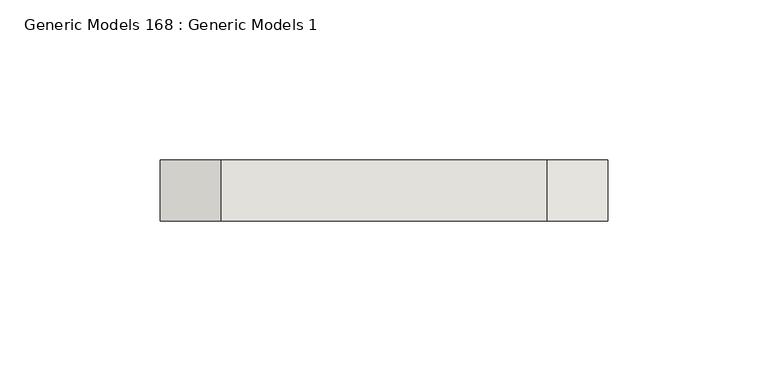
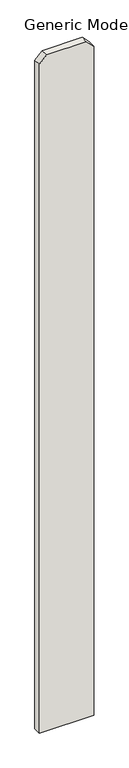
"""IFC4 building model written with IfcOpenShell, lengths in millimetres: wall geometry, Generic Models 168 : Generic Models 1."""

from ifc_helpers import new_model, si_unit, frame, origin, place, context, project, spatial, polyline, outline, extrude, source, transform, mapped, element, save


def generic_models_168_generic_models_1_7be96792(model_context):
    return source(origin(), model_context, "Body", "SweptSolid", [
        extrude(outline(polyline([(76.2, 324585.0125), (1885.95, 324585.0125), (1905.0, 324565.9625), (1905.0, 324464.3625), (1885.95, 324445.3125), (76.2, 324445.3125), (76.2, 324585.0125)])), frame((0.0, 547.6875, 0.0), z_axis=(0.0, 1.0, 0.0), x_axis=(0.0, 0.0, 1.0)), (0.0, 0.0, 1.0), 19.05),
    ])


if __name__ == "__main__":
    model = new_model("IFC4")
    model_context = context("Model", 3, world=origin())
    ifc_project = project(units=[si_unit("LENGTHUNIT", "METRE", prefix="MILLI")], contexts=[model_context])
    site = spatial("IfcSite", under=ifc_project)
    building = spatial("IfcBuilding", under=site)
    placement = place(None, origin())
    generic_models_168_generic_models_1_shape = generic_models_168_generic_models_1_7be96792(model_context)
    element("IfcWall", 1, ObjectType="Generic Models 168 : Generic Models 1", at=placement, inside=building, context=model_context, shape_type="MappedRepresentation", body=[
        mapped(generic_models_168_generic_models_1_shape, transform((0.0, 0.0, 0.0), x_axis=(1.0, 0.0, 0.0), y_axis=(0.0, 1.0, 0.0), z_axis=(0.0, 0.0, 1.0))),
    ])
    save(model, "model.ifc")

# Revit data of these elements
# Element 1 (IfcWall, "Generic Models 168 : Generic Models 1")
#   Materials on its faces: "VERTICAL 1X6 CEDAR PLANKS W/ CLEAR WOOD SEALER"
# Materials
#   "VERTICAL 1X6 CEDAR PLANKS W/ CLEAR WOOD SEALER": class "Wood", colour RGB 234 198 147, transparency 0, Description = "Pinus Echinata", Cost = 0
